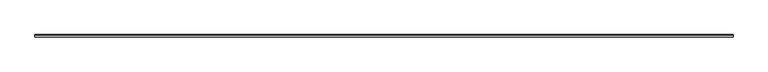
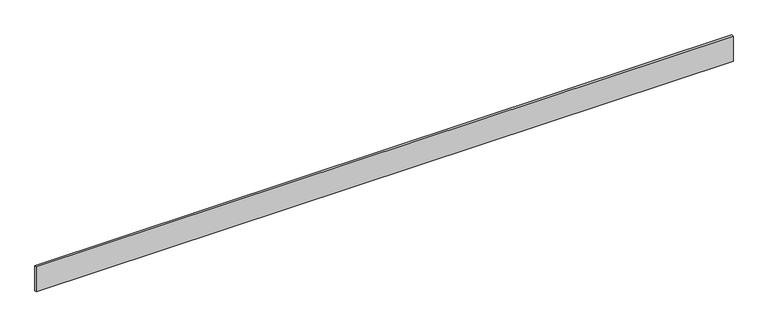
"""IFC4 building model written with IfcOpenShell, lengths in millimetres: proxy geometry, Generic Models 7:Generic Models 1:8:Generic Models 1:8 : Generic Models 7:Generic Models 1:337419:11 : Generic Models 7:Generic Models 1:8:Generic Models 1:8 : Generic Models 7:Generic Models 1:337419:315935."""

from ifc_helpers import new_model, si_unit, frame, origin, place, context, project, spatial, polyline, outline, extrude, source, transform, mapped, element, save


def generic_models_214c4651(model_context):
    return source(origin(), model_context, "Body", "SweptSolid", [
        extrude(outline(polyline([(-568263.8550502, 8757.3617105), (-568263.0438044, 8756.5504648), (-568263.0438044, 8573.2117105), (-568278.9188044, 8573.2117105), (-568278.9188044, 8757.3617105), (-568263.8550502, 8757.3617105)])), frame((591306.0367242, 0.0, 0.0), z_axis=(1.0, 0.0, 0.0), x_axis=(0.0, 1.0, 0.0)), (0.0, 0.0, 1.0), 4876.8),
    ])


if __name__ == "__main__":
    model = new_model("IFC4")
    model_context = context("Model", 3, world=origin())
    ifc_project = project(units=[si_unit("LENGTHUNIT", "METRE", prefix="MILLI")], contexts=[model_context])
    site = spatial("IfcSite", under=ifc_project)
    building = spatial("IfcBuilding", under=site)
    placement = place(None, origin())
    generic_models_shape = generic_models_214c4651(model_context)
    element("IfcBuildingElementProxy", 1, Name="Generic Models 7:Generic Models 1:8:Generic Models 1:8 : Generic Models 7:Generic Models 1:337419:11 : Generic Models 7:Generic Models 1:8:Generic Models 1:8 : Generic Models 7:Generic Models 1:337419:315935", ObjectType="Generic Models 7:Generic Models 1:8:Generic Models 1:8 : Generic Models 7:Generic Models 1:337419:11 : Generic Models 7:Generic Models 1:8:Generic Models 1:8 : Generic Models 7:Generic Models 1:337419:315935", at=placement, inside=building, context=model_context, shape_type="MappedRepresentation", body=[
        mapped(generic_models_shape, transform((0.0, 0.0, 0.0), x_axis=(1.0, 0.0, 0.0), y_axis=(0.0, 1.0, 0.0), z_axis=(0.0, 0.0, 1.0))),
    ])
    save(model, "model.ifc")

# Revit data of these elements
# Type "Generic Models 7:Generic Models 1:8:Generic Models 1:8 : Generic Models 7:Generic Models 1:337419:11 : Generic Models 7:Generic Models 1:8:Generic Models 1:8 : Generic Models 7:Generic Models 1:337419:315935"
#   NameOverride = "Generic Models 7:Generic Models 1:8:Generic Models 1:8 : Generic Models 7:Generic Models 1:337419:315935"
#   ObjectTypeOverride = "Generic Models 1:8 : Generic Models 7:Generic Models 1:337419"
#   Reference = "Generic Models 1"
#   Tag = "315935"
# Element 1 (IfcBuildingElementProxy, "Generic Models 7:Generic Models 1:8:Generic Models 1:8 : Generic Models 7:Generic Models 1:337419:11 : Generic Models 7:Generic Models 1:8:Generic Models 1:8 : Generic Models 7:Generic Models 1:337419:315935")
#   Materials on its faces: "ENGINEERED WOOD TRIM (LP SMARTSIDE)"
# Materials
#   "ENGINEERED WOOD TRIM (LP SMARTSIDE)": class "Wood", colour RGB 108 80 40, transparency 0, Description = "Pinus Echinata", Cost = 0
